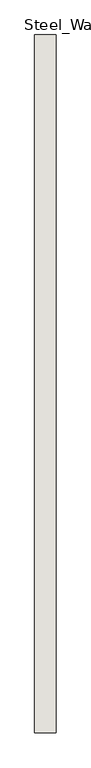
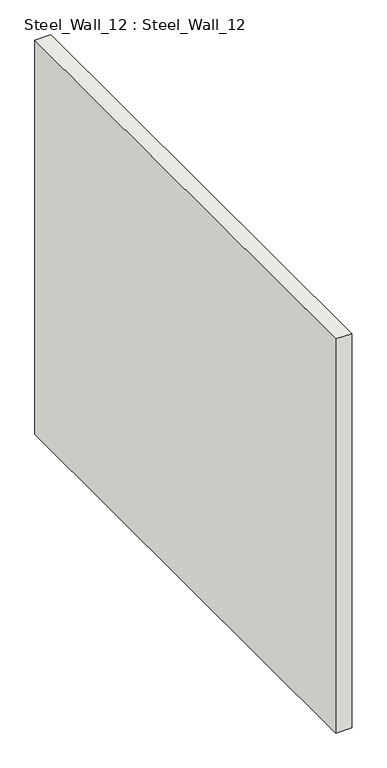
"""IFC4 building model written with IfcOpenShell, lengths in millimetres: wall geometry, Steel_Wall_12 : Steel_Wall_12."""

from ifc_helpers import new_model, si_unit, frame, origin, place, context, project, spatial, polyline, outline, extrude, source, transform, mapped, element, save


def steel_wall_12_steel_wall_12_e47ad89f(model_context):
    return source(origin(), model_context, "Body", "SweptSolid", [
        extrude(outline(polyline([(4785.0, 7415.0), (4785.0, 4165.0), (4685.0, 4165.0), (4685.0, 7415.0), (4785.0, 7415.0)])), frame((0.0, 0.0, 250.0), z_axis=(0.0, 0.0, 1.0), x_axis=(1.0, 0.0, 0.0)), (0.0, 0.0, 1.0), 2600.0),
    ])


if __name__ == "__main__":
    model = new_model("IFC4")
    model_context = context("Model", 3, world=origin())
    ifc_project = project(units=[si_unit("LENGTHUNIT", "METRE", prefix="MILLI")], contexts=[model_context])
    site = spatial("IfcSite", under=ifc_project)
    building = spatial("IfcBuilding", under=site)
    placement = place(None, origin())
    steel_wall_12_steel_wall_12_shape = steel_wall_12_steel_wall_12_e47ad89f(model_context)
    element("IfcWall", 1, ObjectType="Steel_Wall_12 : Steel_Wall_12", at=placement, inside=building, context=model_context, shape_type="MappedRepresentation", body=[
        mapped(steel_wall_12_steel_wall_12_shape, transform((0.0, 0.0, 0.0), x_axis=(1.0, 0.0, 0.0), y_axis=(0.0, 1.0, 0.0), z_axis=(0.0, 0.0, 1.0))),
    ])
    save(model, "model.ifc")

# Revit data of these elements
# Type "Steel_Wall_12 : Steel_Wall_12"
#   NameOverride = "Steel_Wall_12"
# Element 1 (IfcWall, "Steel_Wall_12 : Steel_Wall_12")
#   Materials on its faces: "IfcSurfaceStyle #33"
# Materials
#   "IfcSurfaceStyle #33": class "Unassigned", colour RGB 214 214 214, transparency 0
